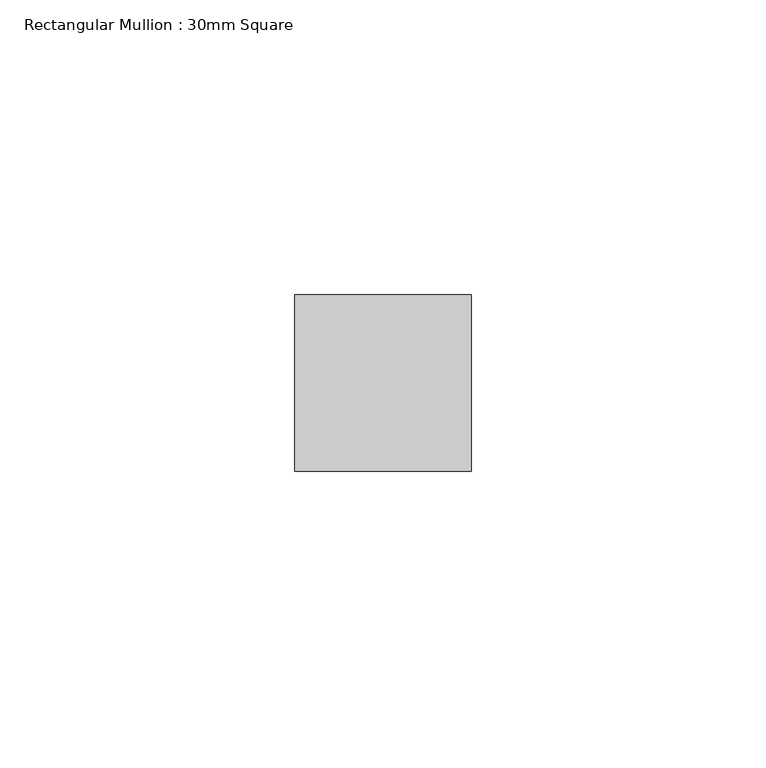
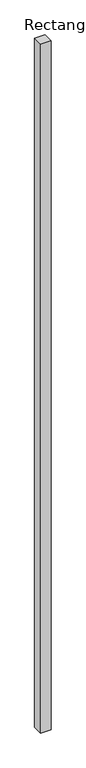
"""IFC4 building model written with IfcOpenShell, lengths in millimetres: member geometry, Rectangular Mullion : 30mm Square."""

from ifc_helpers import new_model, si_unit, frame, origin, place, context, project, spatial, polyline, outline, extrude, source, transform, mapped, element, save


def rectangular_mullion_30mm_square_8e8e927e(model_context):
    return source(origin(), model_context, "Body", "SweptSolid", [
        extrude(outline(polyline([(15.0, 15.0), (15.0, -15.0), (-15.0, -15.0), (-15.0, 15.0), (15.0, 15.0)])), frame((0.0, 0.0, -2083.4347963), z_axis=(0.0, 0.0, 1.0), x_axis=(1.0, 0.0, 0.0)), (0.0, 0.0, 1.0), 2083.4347963),
    ])


if __name__ == "__main__":
    model = new_model("IFC4")
    model_context = context("Model", 3, world=origin())
    ifc_project = project(units=[si_unit("LENGTHUNIT", "METRE", prefix="MILLI")], contexts=[model_context])
    site = spatial("IfcSite", under=ifc_project)
    building = spatial("IfcBuilding", under=site)
    placement = place(None, origin())
    rectangular_mullion_30mm_square_shape = rectangular_mullion_30mm_square_8e8e927e(model_context)
    element("IfcMember", 1, ObjectType="Rectangular Mullion : 30mm Square", at=placement, inside=building, context=model_context, shape_type="MappedRepresentation", body=[
        mapped(rectangular_mullion_30mm_square_shape, transform((0.0, 0.0, 0.0), x_axis=(1.0, 0.0, 0.0), y_axis=(0.0, 1.0, 0.0), z_axis=(0.0, 0.0, 1.0))),
    ])
    save(model, "model.ifc")

# Revit data of these elements
# Type "Rectangular Mullion : 30mm Square"
#   built-in parameter 1007304 = 0.0984252 (stored number, unit not read)
#   built-in parameter 1007301 = 0.0492126 (stored number, unit not read)
#   built-in parameter 1007300 = 0.0492126 (stored number, unit not read)
# Element 1 (IfcMember, "Rectangular Mullion : 30mm Square")
#   Materials on its faces: "Aluminum"
# Materials
#   "Aluminum": class "Metal", colour RGB 244 244 244, transparency 0, Description = "Aluminum 6061", Cost = 0
